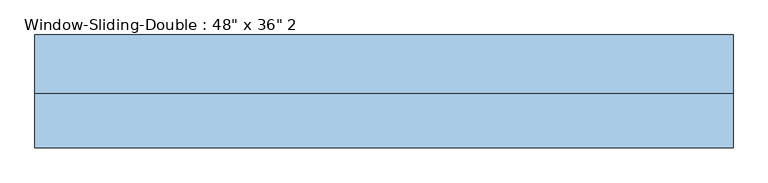
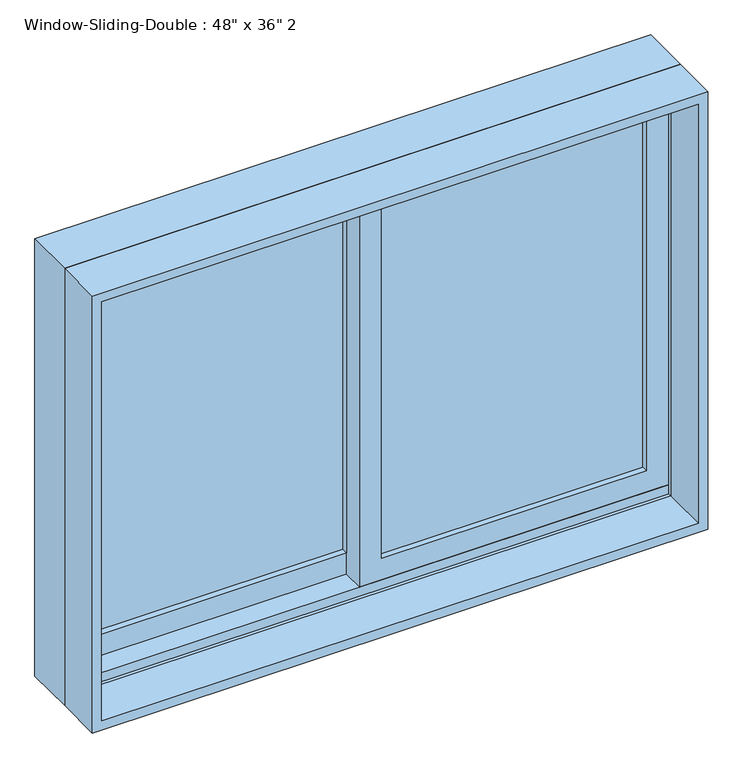
"""IFC4 building model written with IfcOpenShell, lengths in millimetres: window geometry."""

from ifc_helpers import new_model, si_unit, frame, origin, place, context, project, spatial, polyline, outline, extrude, faceted_brep, source, transform, mapped, element, save


def window_4b12ce77(model_context):
    return source(origin(), model_context, "Body", "SolidModel", [
        faceted_brep([(-609.6, 2.54, 914.4), (-609.6, 104.14, 914.4), (609.6, 104.14, 914.4), (609.6, 2.54, 914.4), (-568.6778905, 104.14, 1787.8778905), (-568.6778905, 97.79, 1787.8778905), (-568.6778905, 97.79, 933.45), (-568.6778905, 104.14, 933.45), (568.6778905, 97.79, 1787.8778905), (568.6778905, 97.79, 933.45), (590.55, 97.79, 933.45), (590.55, 97.79, 1809.75), (-590.55, 97.79, 1809.75), (-590.55, 97.79, 933.45), (-590.55, 2.54, 1809.75), (-590.55, 2.54, 933.45), (-590.55, 8.89, 933.45), (-590.55, 8.89, 952.5), (-590.55, 53.34, 952.5), (-590.55, 53.34, 933.45), (609.6, 2.54, 1828.8), (-609.6, 2.54, 1828.8), (590.55, 2.54, 1809.75), (590.55, 2.54, 933.45), (-609.6, 104.14, 1828.8), (609.6, 104.14, 1828.8), (568.6778905, 104.14, 933.45), (568.6778905, 104.14, 1787.8778905), (590.55, 53.34, 933.45), (590.55, 53.34, 952.5), (590.55, 8.89, 952.5), (590.55, 8.89, 933.45)], [[[0, 1, 2, 3]], [[4, 5, 6, 7]], [[5, 8, 9, 10, 11, 12, 13, 6]], [[12, 14, 15, 16, 17, 18, 19, 13]], [[0, 3, 20, 21], [22, 23, 15, 14]], [[24, 1, 0, 21]], [[2, 1, 24, 25], [4, 7, 26, 27]], [[5, 4, 27, 8]], [[12, 11, 22, 14]], [[21, 20, 25, 24]], [[8, 27, 26, 9]], [[22, 11, 10, 28, 29, 30, 31, 23]], [[20, 3, 2, 25]], [[26, 7, 6, 13, 19, 28, 10, 9]], [[28, 19, 18, 29]], [[29, 18, 17, 30]], [[30, 17, 16, 31]], [[15, 23, 31, 16]]]),
        extrude(outline(polyline([(1828.8, -609.6), (914.4, -609.6), (914.4, 609.6), (1828.8, 609.6), (1828.8, -609.6)]), holes=[polyline([(1809.75, 590.55), (933.45, 590.55), (933.45, -590.55), (1809.75, -590.55), (1809.75, 590.55)])]), frame((0.0, -92.71, 0.0), z_axis=(0.0, 1.0, 0.0), x_axis=(0.0, 0.0, 1.0)), (0.0, 0.0, 1.0), 95.25),
        extrude(outline(polyline([(546.1, 40.64), (546.1, 34.29), (22.225, 34.29), (22.225, 40.64), (546.1, 40.64)])), frame((0.0, 0.0, 996.95), z_axis=(0.0, 0.0, 1.0), x_axis=(1.0, 0.0, 0.0)), (0.0, 0.0, 1.0), 768.35),
        extrude(outline(polyline([(546.1, 27.94), (546.1, 21.59), (22.225, 21.59), (22.225, 27.94), (546.1, 27.94)])), frame((0.0, 0.0, 996.95), z_axis=(0.0, 0.0, 1.0), x_axis=(1.0, 0.0, 0.0)), (0.0, 0.0, 1.0), 768.35),
        extrude(outline(polyline([(-22.225, 85.09), (-22.225, 78.74), (-546.1, 78.74), (-546.1, 85.09), (-22.225, 85.09)])), frame((0.0, 0.0, 996.95), z_axis=(0.0, 0.0, 1.0), x_axis=(1.0, 0.0, 0.0)), (0.0, 0.0, 1.0), 768.35),
        extrude(outline(polyline([(-22.225, 72.39), (-22.225, 66.04), (-546.1, 66.04), (-546.1, 72.39), (-22.225, 72.39)])), frame((0.0, 0.0, 996.95), z_axis=(0.0, 0.0, 1.0), x_axis=(1.0, 0.0, 0.0)), (0.0, 0.0, 1.0), 768.35),
        extrude(outline(polyline([(933.45, -590.55), (933.45, 22.225), (1809.75, 22.225), (1809.75, -590.55), (933.45, -590.55)]), holes=[polyline([(1765.3, -22.225), (996.95, -22.225), (996.95, -546.1), (1765.3, -546.1), (1765.3, -22.225)])]), frame((0.0, 53.34, 0.0), z_axis=(0.0, 1.0, 0.0), x_axis=(0.0, 0.0, 1.0)), (0.0, 0.0, 1.0), 44.45),
        extrude(outline(polyline([(952.5, 590.55), (1809.75, 590.55), (1809.75, -22.225), (952.5, -22.225), (952.5, 590.55)]), holes=[polyline([(996.95, 22.225), (1765.3, 22.225), (1765.3, 546.1), (996.95, 546.1), (996.95, 22.225)])]), frame((0.0, 8.89, 0.0), z_axis=(0.0, 1.0, 0.0), x_axis=(0.0, 0.0, 1.0)), (0.0, 0.0, 1.0), 44.45),
    ])


if __name__ == "__main__":
    model = new_model("IFC4")
    model_context = context("Model", 3, world=origin())
    ifc_project = project(units=[si_unit("LENGTHUNIT", "METRE", prefix="MILLI")], contexts=[model_context])
    site = spatial("IfcSite", under=ifc_project)
    building = spatial("IfcBuilding", under=site)
    placement = place(None, origin())
    window_shape = window_4b12ce77(model_context)
    element("IfcWindow", 1, ObjectType="Window-Sliding-Double : 48\" x 36\" 2", at=placement, inside=building, context=model_context, shape_type="MappedRepresentation", body=[
        mapped(window_shape, transform((0.0, 0.0, 0.0), x_axis=(1.0, 0.0, 0.0), y_axis=(0.0, 1.0, 0.0), z_axis=(0.0, 0.0, 1.0))),
    ])
    save(model, "model.ifc")

# Revit data of these elements
# Type "Window-Sliding-Double : 48\" x 36\" 2"
#   Type Mark = "16"
#   Fire Rating = "0.5h"
#   Assembly Code = "B2020100"
#   Analytic Construction = "Double glazing - domestic"
#   Window Inset [instance default] = 0' - 0"
#   Wall Thickness [instance default] = 0' - 6"
#   Visual Light Transmittance = 0.81
#   Thermal Resistance (R) = 0.319569 (m²·K)/W
#   Solar Heat Gain Coefficient = 0.76
#   Muntin Width = 1' - 8 5/8"
#   Muntin Height = 2' - 6 1/4"
#   Interior Wall Closure [instance default] = 0' - 2 3/4"
#   Heat Transfer Coefficient (U) = 3.12929 W/(m²·K)
#   Frame Extension [instance default] = 0' - 0 1/4"
#   Exterior Wall Closure [instance default] = 0' - 1 1/4"
#   Rough Width = 4' - 0 1/2"
#   Rough Height = 3' - 0 1/2"
#   Height = 3' - 0"
#   Extension Jamb [instance default] = 0' - 2 3/4"
#   Default Sill Height = 3' - 0"
#   Width = 4' - 0"
#   Interior Trim Visibility [instance default] = yes
#   Indicator Visibility [instance default] = yes
#   Exterior Trim Visibility [instance default] = yes
#   Muntin Visibility = no
#   Extension Jamb Visibility [instance default] = yes
#   Muntin Pattern = Muntin Pattern_2x2 : Muntin Pattern_2x2
#   Interior Trim Material = Wood - Stained
#   Interior Trim = Trim-Window-Interior-Flat : Picture Frame
#   Interior Frame Material = Wood - Stained
#   Glass Panel Material = Glass
#   Exterior Trim Material = Clad - White
#   Exterior Trim = Trim-Window-Exterior-Flat : with Sill
#   Exterior Frame Material = Clad - White
#   Wall Closure = (empty or 0)
# Element 1 (IfcWindow, "Window-Sliding-Double : 48\" x 36\" 2")
#   Wall Thickness = 0' - 7"
#   Extension Jamb = 0' - 3 3/4"
#   Materials on its faces: "Wood - Stained", "Glass", "Clad - White"
# Materials
#   "Wood - Stained": class "Wood", colour RGB 224 178 126, transparency 0, Cost = 0
#   "Glass": class "Glass", colour RGB 218 227 224, transparency 0.85, Description = "Soda Lime Glass", Cost = 0
#   "Clad - White": class "Wood", colour RGB 242 242 238, transparency 0, Cost = 0
